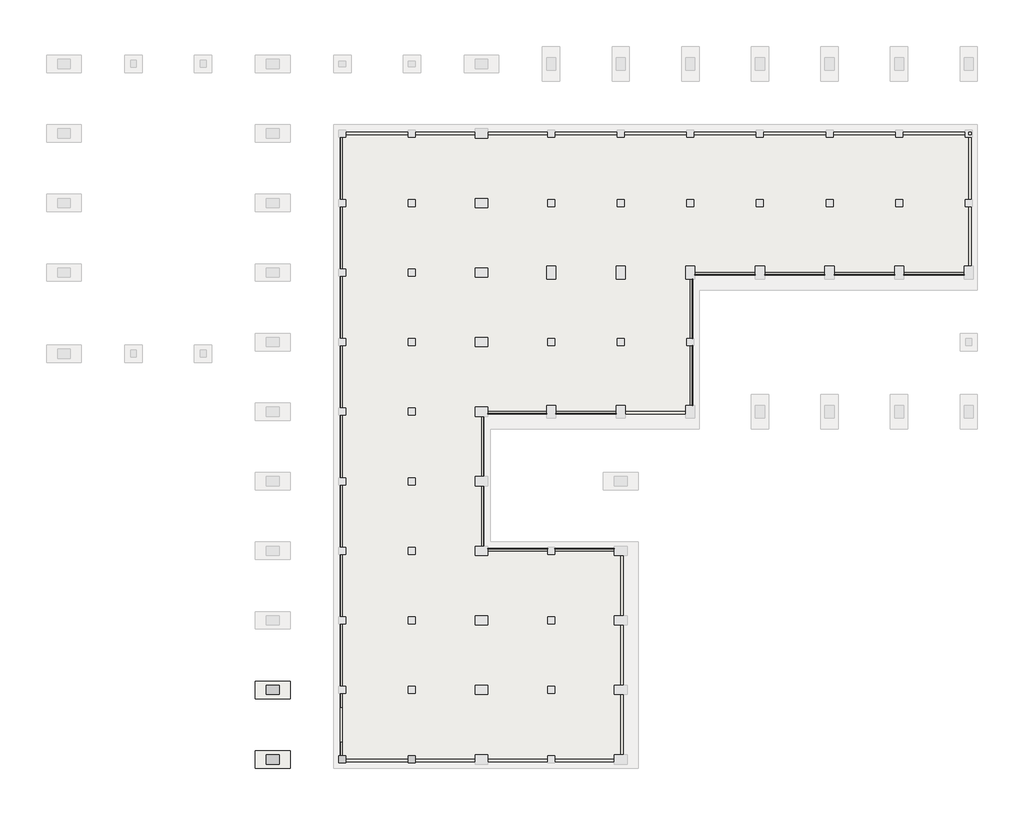
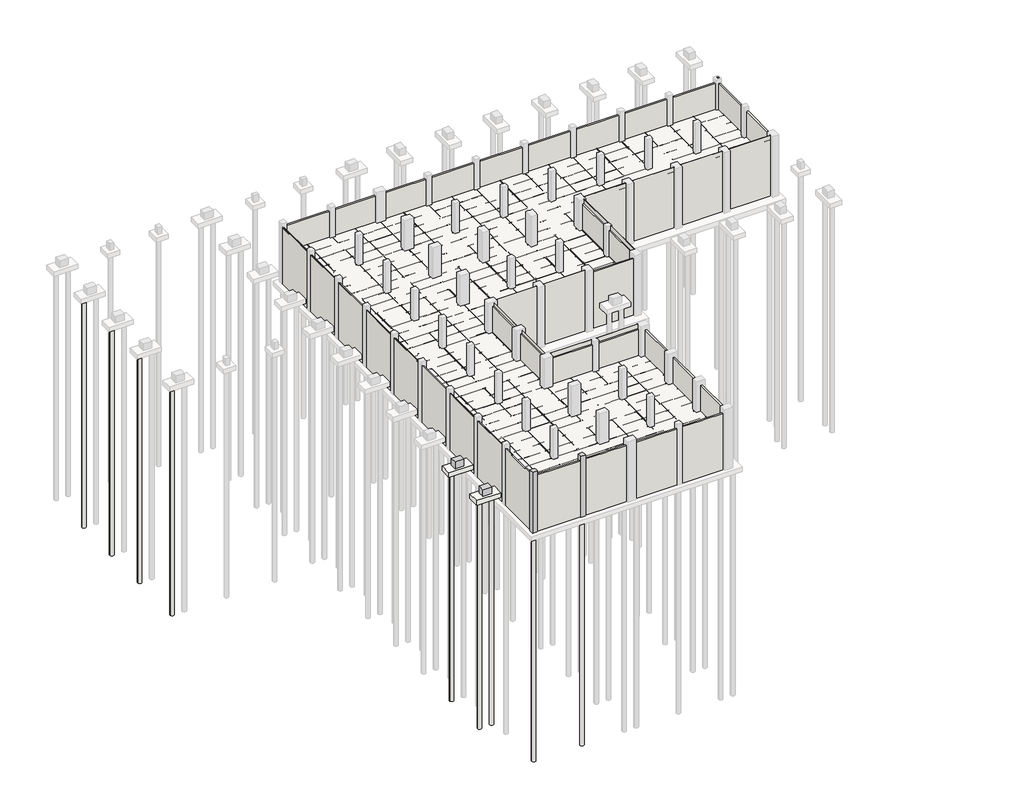
# Not in any storey, part 1 of 16: 12 slabs, 10 walls, 8 beams, 4 columns.
# Revit data of these elements (continued)
# Type "Steel Framing_H_KS : H_SB_AR_S02_H-400x200x8x13_BSG2" (continued)
#   Type Comments = "MAIN"
#   Type Mark = "BSG2"
#   H_SectionID = "H-400x200x8x13"
#   H_Ratio for Additional Steel Plate = 0.2
#   Width = 20.0 cm
#   Web Thickness = 0.8 cm
#   Web Fillet = 1.6 cm
#   Warping Constant = 649000.0 cm⁶
#   Torsional Moment of Inertia = 35.8981 cm⁴
#   Section Area = 84.12 cm²
#   Plastic Modulus weak axis = 268.0 cm³
#   Plastic Modulus strong axis = 1330.0 cm³
#   Perimeter = 1.56 m²/m
#   Nominal Weight = 66.00 kgf/m
#   Moment of Inertia weak axis = 1740.00 cm⁴
#   Moment of Inertia strong axis = 23700.00 cm⁴
#   Height = 40.0 cm
#   Flange Thickness = 1.3 cm
#   Elastic Modulus weak axis = 174.0 cm³
#   Elastic Modulus strong axis = 1190.0 cm³
#   Centroid Vertical = 20.0 cm
#   Centroid Horizontal = 10.0 cm
#   Bolt Spacing = 8.89 cm
#   Length [instance default] = 1500 mm
#   Structural Material [instance default] = Steel, 45-345
#   Section Name Key = ""
#   Assembly Code = ""
# Type "Steel Framing_H_KS : H_SB_AR_S02_H-400x200x8x13_BSB1"
#   Type Comments = "MAIN"
#   Type Mark = "BSB1"
#   H_SectionID = "H-400x200x8x13"
#   H_Ratio for Additional Steel Plate = 0.2
#   Width = 20.0 cm
#   Web Thickness = 0.8 cm
#   Web Fillet = 1.6 cm
#   Warping Constant = 649000.0 cm⁶
#   Torsional Moment of Inertia = 35.8981 cm⁴
#   Section Area = 84.12 cm²
#   Plastic Modulus weak axis = 268.0 cm³
#   Plastic Modulus strong axis = 1330.0 cm³
#   Perimeter = 1.56 m²/m
#   Nominal Weight = 66.00 kgf/m
#   Moment of Inertia weak axis = 1740.00 cm⁴
#   Moment of Inertia strong axis = 23700.00 cm⁴
#   Height = 40.0 cm
#   Flange Thickness = 1.3 cm
#   Elastic Modulus weak axis = 174.0 cm³
#   Elastic Modulus strong axis = 1190.0 cm³
#   Centroid Vertical = 20.0 cm
#   Centroid Horizontal = 10.0 cm
#   Bolt Spacing = 8.89 cm
#   Length [instance default] = 1500 mm
#   Structural Material [instance default] = Steel, 45-345
#   Section Name Key = ""
#   Assembly Code = ""
# Type "Steel Framing_C_KS : H_SB_AR_S02_C-150x75x6.5x10_J1"
#   Type Mark = "J1"
#   H_SectionID = "C-150x75x6.5x10"
#   Assembly Code = "B10"
#   H_Ratio for Additional Steel Plate = 0.2
#   Perimeter = 0.51 m²/m
#   Nominal Weight = 18.60 kgf/m
#   Length [instance default] = 1000 mm
#   bf = 75 mm
#   d = 150 mm
#   tf = 10 mm
#   tw = 6.5 mm
#   x = 22.8 mm
#   A = 0.002371 m²
#   Structural Material [instance default] = Steel, 45-345
# Type "RC_Column_Rectangular : H_SC_AR_S15_UG PED_Bit_800x1100_PD1"
#   Type Mark = "PD1"
#   Type Comments = "UG"
#   H_SectionID = "600 x 900"
#   H_Rebar Ratio = 0.3
#   Width = 800 mm
#   Depth = 1100 mm
#   hec_material3 [instance default] = none
#   hec_material2 [instance default] = none
#   hec_material1 [instance default] = none
#   Structural Material [instance default] = none
#   Description = (empty or 0)
# Type "RC_Column_Rectangular : H_SC_AR_S15_UG PED_Bit_600x600_BC1"
#   Type Mark = "BC1"
#   Type Comments = "UG"
#   H_SectionID = "600 x 600"
#   H_Rebar Ratio = 0.3
#   Width = 600 mm
#   Depth = 600 mm
#   hec_material3 [instance default] = none
#   hec_material2 [instance default] = none
#   hec_material1 [instance default] = none
#   Structural Material [instance default] = none
#   Description = (empty or 0)
# Type "H_FL_AR_S05_Grating_T32_B FL"
#   Keynote = ""
#   Type Comments = ""
#   Description = ""
#   Function = 1
#   Layers, outside or top first: 32 mm "Grating(1)" (function 4)
# Type "Foundation Rectangular (Non-Pile) : H_SF_AR_S18_Shallow Fdn_Bitumen_1500x3000xT600_F1"
#   Type Comments = "UG"
#   Type Mark = "F1"
#   Top bar = "D25@300"
#   Description = "UG Shallow Foundation"
#   Bottom bar = "D20@300"
#   H_Rebar Ratio = 0.12
#   Width = 1500 mm
#   Length = 3000 mm
#   Foundation Thickness = 600 mm
#   Structural Material [instance default] = none
#   Assembly Code = ""
# Type "PILE : H_SF_AR_S19_PHC Pile_Pre-boring_D500_L30"
#   Assembly Code = "A1020120"
#   반지름 = 250 mm
#   최소 내포 = 150 mm
#   Diameter = 500 mm
#   Depth = 30000 mm
#   Structural Material [instance default] = none
# Type "H_WA_AR_B02_Ext Wall_RC_UG_Bitumen_T200_W1"
#   Type Comments = "UG"
#   Type Mark = "W1"
#   H_Rebar Ratio = 0.12
#   Layers, outside or top first: 200 mm "00_Concrete_Reinf. Conc." (function 1)
# Element 1 (IfcBeam, "Steel Framing_H_KS : H_SB_AR_S02_H-400x200x8x13_BSG2")
#   Structural Material = Steel, 45-345
#   Phase Created = New Construction
#   Materials on its faces: "Steel, 45-345"
# Element 2 (IfcBeam, "Steel Framing_H_KS : H_SB_AR_S02_H-400x200x8x13_BSB1")
#   Structural Material = Steel, 45-345
#   Phase Created = New Construction
#   Materials on its faces: "Steel, 45-345"
# Elements 3, 4, 5, 6, 7, 8 (IfcBeam, "Steel Framing_C_KS : H_SB_AR_S02_C-150x75x6.5x10_J1")
#   Structural Material = Steel, 45-345
#   Phase Created = New Construction
#   Materials on its faces: "Steel, 45-345"
# Elements 9, 10 (IfcColumn, "RC_Column_Rectangular : H_SC_AR_S15_UG PED_Bit_800x1100_PD1")
#   Comments = ""
#   hec_material3 = none
#   hec_material2 = none
#   hec_material1 = none
#   Structural Material = 00_Concrete_Reinf. Conc.
#   Phase Created = New Construction
#   Materials on its faces: "00_Concrete_Reinf. Conc."
# Elements 11, 12 (IfcColumn, "RC_Column_Rectangular : H_SC_AR_S15_UG PED_Bit_600x600_BC1")
#   Comments = ""
#   hec_material3 = none
#   hec_material2 = none
#   hec_material1 = none
#   Structural Material = 00_Concrete_Reinf. Conc.
#   Phase Created = New Construction
#   Materials on its faces: "00_Concrete_Reinf. Conc."
# Element 13 (IfcSlab, "H_FL_AR_S05_Grating_T32_B FL")
#   Height Offset From Level = 0 mm
#   Phase Created = New Construction
#   Materials on its faces: "Grating(1)"
# Elements 14, 15 (IfcSlab, "Foundation Rectangular (Non-Pile) : H_SF_AR_S18_Shallow Fdn_Bitumen_1500x3000xT600_F1")
#   Comments = ""
#   Structural Material = 00_Concrete_Reinf. Conc.
#   Phase Created = New Construction
#   Materials on its faces: "00_Concrete_Reinf. Conc."
# Elements 16, 17, 18, 19, 20, 21, 22 (IfcSlab, "PILE : H_SF_AR_S19_PHC Pile_Pre-boring_D500_L30")
#   Structural Material = Concrete, Precast
#   Phase Created = New Construction
#   Materials on its faces: "Concrete, Precast"
# Elements 23, 24 (IfcSlab, "PILE : H_SF_AR_S19_PHC Pile_Pre-boring_D500_L30")
#   Structural Material = none
#   Phase Created = New Construction
# Element 25 (IfcWall, "H_WA_AR_B02_Ext Wall_RC_UG_Bitumen_T200_W1")
#   Top Offset = -500 mm
#   Base Offset = 0 mm
#   wall height = 7500 mm
#   Phase Created = New Construction
#   Base Constraint = TOC B2
#   Top Constraint = TOF GF
#   Materials on its faces: "00_Concrete_Reinf. Conc."
# Elements 26, 27, 28, 29, 30, 31, 32, 33, 34 (IfcWall, "H_WA_AR_B02_Ext Wall_RC_UG_Bitumen_T200_W1")
#   Top Offset = 0 mm
#   Base Offset = 0 mm
#   wall height = 8000 mm
#   Phase Created = New Construction
#   Base Constraint = TOC B2
#   Top Constraint = TOF GF
#   Materials on its faces: "00_Concrete_Reinf. Conc."
# Materials
#   "Steel, 45-345": class "Metal", colour RGB 189 187 185, transparency 0, Description = "Steel 345 MPa", Cost = 0
#   "Grating(1)": class "Generic", colour RGB 120 120 120, transparency 0, Description = "GRATING", Cost = 0
#   "00_Concrete_Reinf. Conc.": class "Concrete", colour RGB 176 176 176, transparency 0, Description = "Reinf. Conc.", Cost = 0, Image = Concrete.Cast-In-Place.Flat.Polished.Grey.jpg
#   "Concrete, Precast": class "Concrete", colour RGB 115 116 108, transparency 0, Description = "Precast concrete", Cost = 0
